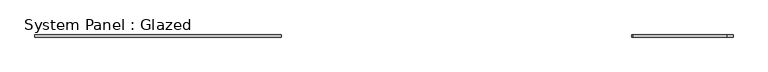
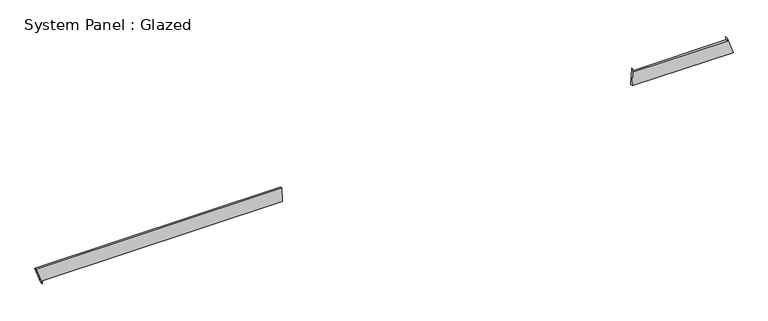
"""IFC4 building model written with IfcOpenShell, lengths in millimetres: plate geometry, System Panel : Glazed."""

import ifcopenshell
import ifcopenshell.guid

model = None  # the IFC model being written
_history = None  # IfcOwnerHistory: only IFC2X3 demands one
_inside = {}  # id of a spatial element -> (the spatial element, [elements in it])
_under = {}  # id of a project, library or spatial element -> (it, [spatial elements below it])
_declared = {}  # id of a project -> (the project, [libraries it declares])
_typed = {}  # id of a type object -> (the type object, [elements of that type])
_made_of = {}  # id of a material, layer set ... -> (it, [elements and type objects made of it])


def new_model(schema):
    """Start an empty IFC model of exactly this schema.

    Asked for "IFC4X3", IfcOpenShell would pick the latest addendum, in which some entities
    have other attributes; the version numbers below select the first issue.
    IFC2X3 requires an IfcOwnerHistory on every rooted entity: one is made here for all.
    """
    global model, _history
    if schema == "IFC4X3":
        model = ifcopenshell.file(schema_version=(4, 3, 0, 0))
    else:
        model = ifcopenshell.file(schema=schema)
    _inside.clear()
    _under.clear()
    _declared.clear()
    _typed.clear()
    _made_of.clear()
    _history = None
    if model.schema == "IFC2X3":
        org = make("IfcOrganization", Name="unknown")
        user = make(
            "IfcPersonAndOrganization",
            ThePerson=make("IfcPerson", FamilyName="unknown"),
            TheOrganization=org,
        )
        app = make(
            "IfcApplication",
            ApplicationDeveloper=org,
            Version="unknown",
            ApplicationFullName="unknown",
            ApplicationIdentifier="unknown",
        )
        _history = make(
            "IfcOwnerHistory",
            OwningUser=user,
            OwningApplication=app,
            ChangeAction="ADDED",
            CreationDate=0,
        )
    return model


def make(cls, **values):
    """One entity of the class cls with the attributes given. An attribute that is None is left unset."""
    return model.create_entity(
        cls, **{name: value for name, value in values.items() if value is not None}
    )


def rooted(cls, **values):
    """An entity with a GlobalId (a new one), such as an element, a storey or a relation."""
    return make(cls, GlobalId=ifcopenshell.guid.new(), OwnerHistory=_history, **values)


def si_unit(unit_type, name, prefix=None):
    """IfcSIUnit, for example si_unit("LENGTHUNIT", "METRE", prefix="MILLI")."""
    return make("IfcSIUnit", UnitType=unit_type, Prefix=prefix, Name=name)


def assignment(units):
    """IfcUnitAssignment: the units of a project."""
    return None if units is None else make("IfcUnitAssignment", Units=units)


def point(xyz):
    """IfcCartesianPoint."""
    return None if xyz is None else make("IfcCartesianPoint", Coordinates=xyz)


def direction(xyz):
    """IfcDirection."""
    return None if xyz is None else make("IfcDirection", DirectionRatios=xyz)


def frame(location, z_axis=None, x_axis=None):
    """IfcAxis2Placement3D, a coordinate frame: its origin and axes. An axis left out is left unset."""
    return make(
        "IfcAxis2Placement3D",
        Location=point(location),
        Axis=direction(z_axis),
        RefDirection=direction(x_axis),
    )


def origin():
    """The frame at (0, 0, 0) with its axes left unset."""
    return frame((0.0, 0.0, 0.0))


def place(relative_to, where):
    """IfcLocalPlacement: puts the frame where relative to a parent placement (None: the world)."""
    return make(
        "IfcLocalPlacement", PlacementRelTo=relative_to, RelativePlacement=where
    )


def context(
    kind, dimensions, precision=None, world=None, true_north=None, identifier=None
):
    """IfcGeometricRepresentationContext, for example the 3D "Model" context."""
    return make(
        "IfcGeometricRepresentationContext",
        ContextIdentifier=identifier,
        ContextType=kind,
        CoordinateSpaceDimension=dimensions,
        Precision=precision,
        WorldCoordinateSystem=world,
        TrueNorth=true_north,
    )


def project(units=None, contexts=None):
    """IfcProject with its units and contexts."""
    return rooted(
        "IfcProject",
        Name="project",
        RepresentationContexts=contexts,
        UnitsInContext=assignment(units),
    )


def spatial(cls, under=None, at=None, **own):
    """A site, building, storey or space (cls), placed at a placement, below another one or the project."""
    s = rooted(cls, ObjectPlacement=at, **own)
    if under is not None:
        _under.setdefault(under.id(), (under, []))[1].append(s)
    return s


def polyline(points):
    """IfcPolyline through the points."""
    return make("IfcPolyline", Points=[point(p) for p in points])


def outline(outer, holes=None, kind="AREA"):
    """IfcArbitraryClosedProfileDef: a profile drawn as a closed curve; with holes, ...WithVoids."""
    if holes is None:
        return make("IfcArbitraryClosedProfileDef", ProfileType=kind, OuterCurve=outer)
    return make(
        "IfcArbitraryProfileDefWithVoids",
        ProfileType=kind,
        OuterCurve=outer,
        InnerCurves=holes,
    )


def extrude(swept, where, along, depth):
    """IfcExtrudedAreaSolid: the profile swept, set in the frame where, extruded along a direction by depth."""
    return make(
        "IfcExtrudedAreaSolid",
        SweptArea=swept,
        Position=where,
        ExtrudedDirection=direction(along),
        Depth=depth,
    )


def shape(context_of_items, identifier, shape_type, items):
    """IfcShapeRepresentation: the items that make up one representation, for example the "Body"."""
    return make(
        "IfcShapeRepresentation",
        ContextOfItems=context_of_items,
        RepresentationIdentifier=identifier,
        RepresentationType=shape_type,
        Items=items,
    )


def source(mapping_origin, context_of_items, identifier, shape_type, items):
    """IfcRepresentationMap: a shape defined once, which mapped items show again and again."""
    return make(
        "IfcRepresentationMap",
        MappingOrigin=mapping_origin,
        MappedRepresentation=shape(context_of_items, identifier, shape_type, items),
    )


def transform(
    local_origin,
    x_axis=None,
    y_axis=None,
    z_axis=None,
    scale=None,
    scale2=None,
    scale3=None,
    uniform=True,
):
    """IfcCartesianTransformationOperator3D, or its non-uniform kind. x_axis, y_axis, z_axis: its Axis1, 2, 3."""
    if uniform:
        return make(
            "IfcCartesianTransformationOperator3D",
            Axis1=direction(x_axis),
            Axis2=direction(y_axis),
            LocalOrigin=point(local_origin),
            Scale=scale,
            Axis3=direction(z_axis),
        )
    return make(
        "IfcCartesianTransformationOperator3DnonUniform",
        Axis1=direction(x_axis),
        Axis2=direction(y_axis),
        LocalOrigin=point(local_origin),
        Scale=scale,
        Axis3=direction(z_axis),
        Scale2=scale2,
        Scale3=scale3,
    )


def mapped(mapping_source, mapping_target):
    """IfcMappedItem: shows the shape of a source again, moved by a transform."""
    return make(
        "IfcMappedItem", MappingSource=mapping_source, MappingTarget=mapping_target
    )


def made_of(thing, what):
    """Note that an element or type object is made of a material, layer set ...; save() writes the relation."""
    if what is not None:
        _made_of.setdefault(what.id(), (what, []))[1].append(thing)
    return thing


def element(
    cls,
    number,
    at=None,
    inside=None,
    cuts=None,
    type_object=None,
    material=None,
    context=None,
    identifier="Body",
    shape_type=None,
    held_by="IfcProductDefinitionShape",
    body=None,
    shapes=None,
    **own,
):
    """One element of the class cls, such as IfcWall. Its Tag is "e" and its number.

    at: its placement. inside: the storey or other place that contains it. cuts: it is an
    opening in that element (IfcRelVoidsElement). A single representation is given by context,
    identifier, shape_type and body (its items); several are given by shapes. held_by: the class
    of the entity that holds the representations. save() writes the other relations.
    """
    e = rooted(cls, Tag="e%d" % number, ObjectPlacement=at, **own)
    if body is not None:
        shapes = [shape(context, identifier, shape_type, body)]
    if shapes is not None:
        e.Representation = make(held_by, Representations=shapes)
    if inside is not None:
        _inside.setdefault(inside.id(), (inside, []))[1].append(e)
    if cuts is not None:
        rooted(
            "IfcRelVoidsElement", RelatingBuildingElement=cuts, RelatedOpeningElement=e
        )
    if type_object is not None:
        _typed.setdefault(type_object.id(), (type_object, []))[1].append(e)
    return made_of(e, material)


def aggregate(whole, parts):
    """IfcRelAggregates: a whole, such as a stair, and the parts it consists of."""
    return rooted("IfcRelAggregates", RelatingObject=whole, RelatedObjects=parts)


def save(model, path):
    """Write the relations noted so far, then the file.

    IfcRelAggregates (storeys below a building ...), IfcRelContainedInSpatialStructure (elements
    in a storey), IfcRelDefinesByType, IfcRelAssociatesMaterial and IfcRelDeclares: one each for
    every whole, place, type object, material and project.
    """
    for whole, parts in _under.values():
        aggregate(whole, parts)
    for where, things in _inside.values():
        rooted(
            "IfcRelContainedInSpatialStructure",
            RelatedElements=things,
            RelatingStructure=where,
        )
    for kind, things in _typed.values():
        rooted("IfcRelDefinesByType", RelatedObjects=things, RelatingType=kind)
    for what, things in _made_of.values():
        rooted("IfcRelAssociatesMaterial", RelatedObjects=things, RelatingMaterial=what)
    for by, libraries in _declared.values():
        rooted("IfcRelDeclares", RelatingContext=by, RelatedDefinitions=libraries)
    model.write(path)


def system_panel_glazed_9f0471fb(model_context):
    return source(origin(), model_context, "Body", "SweptSolid", [
        extrude(outline(polyline([(35.3553391, 2859.8495797), (35.3553391, 4027.1832678), (235.4605257, 3957.794267), (200.1051866, 3957.7948933), (200.0858758, 2867.7205954), (235.4412148, 2867.7199691), (35.3553391, 2859.8495797)])), frame((0.0, -49.5, 0.0), z_axis=(0.0, 1.0, 0.0), x_axis=(0.0, 0.0, 1.0)), (0.0, 0.0, 1.0), 25.0),
        extrude(outline(polyline([(0.0, -3957.4553629), (35.3553391, -3957.4553629), (35.3553391, -1184.8268191), (200.0140372, -1187.4748261), (199.9637313, -4027.1832678), (0.0, -3957.4553629)])), frame((0.0, -49.5, 0.0), z_axis=(0.0, 1.0, 0.0), x_axis=(0.0, 0.0, 1.0)), (0.0, 0.0, 1.0), 25.0),
    ])


if __name__ == "__main__":
    model = new_model("IFC4")
    model_context = context("Model", 3, world=origin())
    ifc_project = project(units=[si_unit("LENGTHUNIT", "METRE", prefix="MILLI")], contexts=[model_context])
    site = spatial("IfcSite", under=ifc_project)
    building = spatial("IfcBuilding", under=site)
    placement = place(None, origin())
    system_panel_glazed_shape = system_panel_glazed_9f0471fb(model_context)
    element("IfcPlate", 1, ObjectType="System Panel : Glazed", at=placement, inside=building, context=model_context, shape_type="MappedRepresentation", body=[
        mapped(system_panel_glazed_shape, transform((0.0, 0.0, 0.0), x_axis=(1.0, 0.0, 0.0), y_axis=(0.0, 1.0, 0.0), z_axis=(0.0, 0.0, 1.0))),
    ])
    save(model, "model.ifc")

# Revit data of these elements
# Element 1 (IfcPlate, "System Panel : Glazed")
#   Materials on its faces: "Glass"
# Materials
#   "Glass": class "Glass", colour RGB 218 227 224, transparency 0.85, Description = "Soda Lime Glass", Cost = 0
